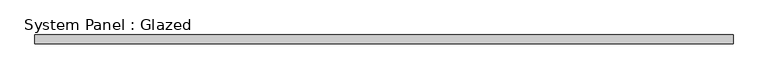
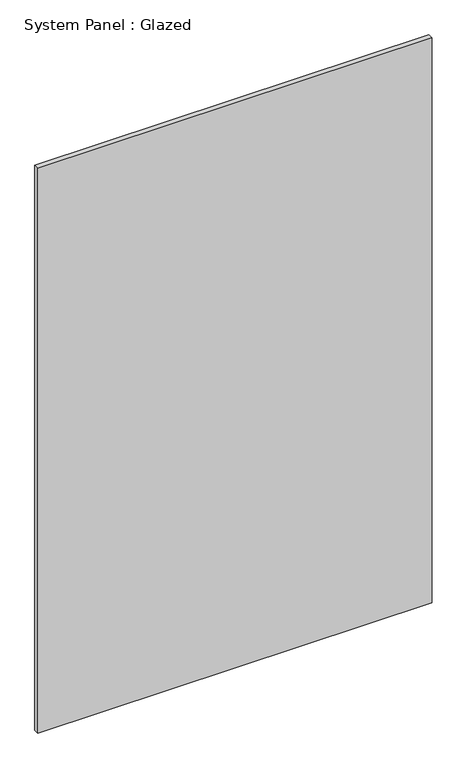
"""IFC4 building model written with IfcOpenShell, lengths in millimetres: plate geometry, System Panel : Glazed."""

from ifc_helpers import new_model, si_unit, origin, origin_with_axes, place, context, project, spatial, polyline, outline, extrude, source, transform, mapped, element, save


def system_panel_glazed_2cf92cf8(model_context):
    return source(origin(), model_context, "Body", "SweptSolid", [
        extrude(outline(polyline([(974.1833333, 24.5), (-974.1833333, 24.5), (-974.1833333, 49.5), (974.1833333, 49.5), (974.1833333, 24.5)])), origin_with_axes(), (0.0, 0.0, 1.0), 2950.0),
    ])


if __name__ == "__main__":
    model = new_model("IFC4")
    model_context = context("Model", 3, world=origin())
    ifc_project = project(units=[si_unit("LENGTHUNIT", "METRE", prefix="MILLI")], contexts=[model_context])
    site = spatial("IfcSite", under=ifc_project)
    building = spatial("IfcBuilding", under=site)
    placement = place(None, origin())
    system_panel_glazed_shape = system_panel_glazed_2cf92cf8(model_context)
    element("IfcPlate", 1, ObjectType="System Panel : Glazed", at=placement, inside=building, context=model_context, shape_type="MappedRepresentation", body=[
        mapped(system_panel_glazed_shape, transform((0.0, 0.0, 0.0), x_axis=(1.0, 0.0, 0.0), y_axis=(0.0, 1.0, 0.0), z_axis=(0.0, 0.0, 1.0))),
    ])
    save(model, "model.ifc")

# Revit data of these elements
# Element 1 (IfcPlate, "System Panel : Glazed")
#   Materials on its faces: "Glass"
# Materials
#   "Glass": class "Glass", colour RGB 0 128 192, transparency 0.9
